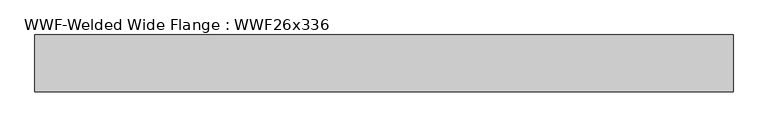
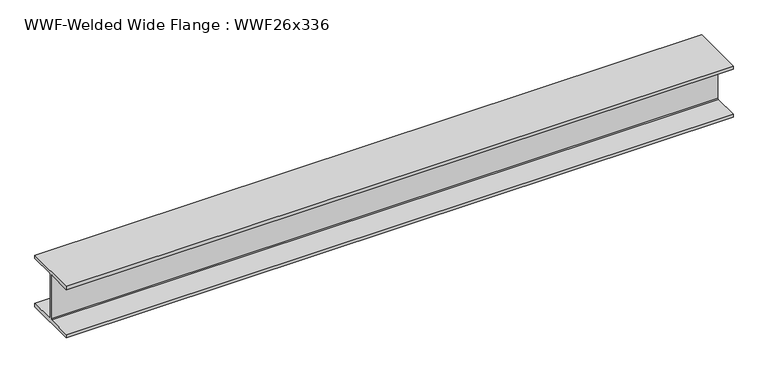
"""IFC4 building model written with IfcOpenShell, lengths in millimetres: beam geometry, WWF-Welded Wide Flange : WWF26x336."""

from ifc_helpers import new_model, si_unit, frame, origin, place, context, project, spatial, polyline, outline, extrude, source, transform, mapped, element, save


def wwf_welded_wide_flange_wwf26x336_68bbe196(model_context):
    return source(origin(), model_context, "Body", "SweptSolid", [
        extrude(outline(polyline([(324.993, -284.988), (324.993, -324.993), (-324.993, -324.993), (-324.993, -284.988), (-20.6375, -284.988), (-9.9949, -274.3454), (-9.9949, 274.3454), (-20.6375, 284.988), (-324.993, 284.988), (-324.993, 324.993), (324.993, 324.993), (324.993, 284.988), (20.6375, 284.988), (9.9949, 274.3454), (9.9949, -274.3454), (20.6375, -284.988), (324.993, -284.988)])), frame((-3827.7582557, 0.0, 0.0), z_axis=(1.0, 0.0, 0.0), x_axis=(0.0, 1.0, 0.0)), (0.0, 0.0, 1.0), 7985.2394153),
    ])


if __name__ == "__main__":
    model = new_model("IFC4")
    model_context = context("Model", 3, world=origin())
    ifc_project = project(units=[si_unit("LENGTHUNIT", "METRE", prefix="MILLI")], contexts=[model_context])
    site = spatial("IfcSite", under=ifc_project)
    building = spatial("IfcBuilding", under=site)
    placement = place(None, origin())
    wwf_welded_wide_flange_wwf26x336_shape = wwf_welded_wide_flange_wwf26x336_68bbe196(model_context)
    element("IfcBeam", 1, ObjectType="WWF-Welded Wide Flange : WWF26x336", at=placement, inside=building, context=model_context, shape_type="MappedRepresentation", body=[
        mapped(wwf_welded_wide_flange_wwf26x336_shape, transform((0.0, 0.0, 0.0), x_axis=(1.0, 0.0, 0.0), y_axis=(0.0, 1.0, 0.0), z_axis=(0.0, 0.0, 1.0))),
    ])
    save(model, "model.ifc")

# Revit data of these elements
# Type "WWF-Welded Wide Flange : WWF26x336"
#   Assembly Code = "B10"
#   Nominal d = "12"
#   W = 336
#   Length [instance default] = 1524 mm
#   bf = 649.986 mm
#   d = 649.986 mm
#   k = 20.638 mm
#   tf = 40.005 mm
#   tw = 19.99 mm
#   A = 0.0635483 m²
#   Structural Material [instance default] = Steel ASTM A572
# Element 1 (IfcBeam, "WWF-Welded Wide Flange : WWF26x336")
#   Structural Material = Metal - Steel 43-275
#   Materials on its faces: "Metal - Steel 43-275"
# Materials
#   "Steel ASTM A572": class "Metal", colour RGB 247 247 247, transparency 0, Description = "Structural steel, high strength low alloy, ASTM - A572 - 50", Cost = 0
#   "Metal - Steel 43-275": class "Metal", colour RGB 247 247 247, transparency 0, Cost = 0
